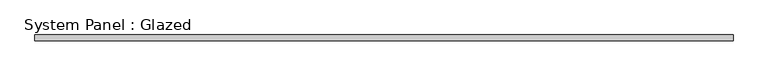
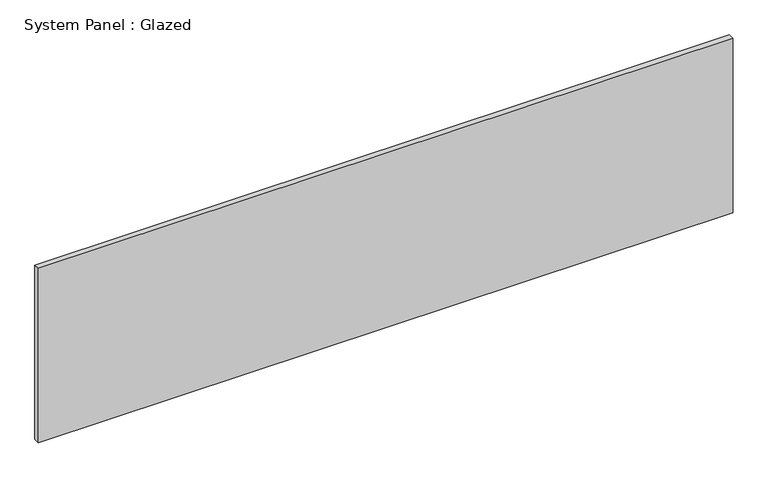
"""IFC4 building model written with IfcOpenShell, lengths in millimetres: plate geometry, System Panel : Glazed."""

import ifcopenshell
import ifcopenshell.guid

model = None  # the IFC model being written
_history = None  # IfcOwnerHistory: only IFC2X3 demands one
_inside = {}  # id of a spatial element -> (the spatial element, [elements in it])
_under = {}  # id of a project, library or spatial element -> (it, [spatial elements below it])
_declared = {}  # id of a project -> (the project, [libraries it declares])
_typed = {}  # id of a type object -> (the type object, [elements of that type])
_made_of = {}  # id of a material, layer set ... -> (it, [elements and type objects made of it])


def new_model(schema):
    """Start an empty IFC model of exactly this schema.

    Asked for "IFC4X3", IfcOpenShell would pick the latest addendum, in which some entities
    have other attributes; the version numbers below select the first issue.
    IFC2X3 requires an IfcOwnerHistory on every rooted entity: one is made here for all.
    """
    global model, _history
    if schema == "IFC4X3":
        model = ifcopenshell.file(schema_version=(4, 3, 0, 0))
    else:
        model = ifcopenshell.file(schema=schema)
    _inside.clear()
    _under.clear()
    _declared.clear()
    _typed.clear()
    _made_of.clear()
    _history = None
    if model.schema == "IFC2X3":
        org = make("IfcOrganization", Name="unknown")
        user = make(
            "IfcPersonAndOrganization",
            ThePerson=make("IfcPerson", FamilyName="unknown"),
            TheOrganization=org,
        )
        app = make(
            "IfcApplication",
            ApplicationDeveloper=org,
            Version="unknown",
            ApplicationFullName="unknown",
            ApplicationIdentifier="unknown",
        )
        _history = make(
            "IfcOwnerHistory",
            OwningUser=user,
            OwningApplication=app,
            ChangeAction="ADDED",
            CreationDate=0,
        )
    return model


def make(cls, **values):
    """One entity of the class cls with the attributes given. An attribute that is None is left unset."""
    return model.create_entity(
        cls, **{name: value for name, value in values.items() if value is not None}
    )


def rooted(cls, **values):
    """An entity with a GlobalId (a new one), such as an element, a storey or a relation."""
    return make(cls, GlobalId=ifcopenshell.guid.new(), OwnerHistory=_history, **values)


def si_unit(unit_type, name, prefix=None):
    """IfcSIUnit, for example si_unit("LENGTHUNIT", "METRE", prefix="MILLI")."""
    return make("IfcSIUnit", UnitType=unit_type, Prefix=prefix, Name=name)


def assignment(units):
    """IfcUnitAssignment: the units of a project."""
    return None if units is None else make("IfcUnitAssignment", Units=units)


def point(xyz):
    """IfcCartesianPoint."""
    return None if xyz is None else make("IfcCartesianPoint", Coordinates=xyz)


def direction(xyz):
    """IfcDirection."""
    return None if xyz is None else make("IfcDirection", DirectionRatios=xyz)


def frame(location, z_axis=None, x_axis=None):
    """IfcAxis2Placement3D, a coordinate frame: its origin and axes. An axis left out is left unset."""
    return make(
        "IfcAxis2Placement3D",
        Location=point(location),
        Axis=direction(z_axis),
        RefDirection=direction(x_axis),
    )


def origin():
    """The frame at (0, 0, 0) with its axes left unset."""
    return frame((0.0, 0.0, 0.0))


def origin_with_axes():
    """The frame at (0, 0, 0) with the z axis (0, 0, 1) and the x axis (1, 0, 0) written out."""
    return frame((0.0, 0.0, 0.0), z_axis=(0.0, 0.0, 1.0), x_axis=(1.0, 0.0, 0.0))


def place(relative_to, where):
    """IfcLocalPlacement: puts the frame where relative to a parent placement (None: the world)."""
    return make(
        "IfcLocalPlacement", PlacementRelTo=relative_to, RelativePlacement=where
    )


def context(
    kind, dimensions, precision=None, world=None, true_north=None, identifier=None
):
    """IfcGeometricRepresentationContext, for example the 3D "Model" context."""
    return make(
        "IfcGeometricRepresentationContext",
        ContextIdentifier=identifier,
        ContextType=kind,
        CoordinateSpaceDimension=dimensions,
        Precision=precision,
        WorldCoordinateSystem=world,
        TrueNorth=true_north,
    )


def project(units=None, contexts=None):
    """IfcProject with its units and contexts."""
    return rooted(
        "IfcProject",
        Name="project",
        RepresentationContexts=contexts,
        UnitsInContext=assignment(units),
    )


def spatial(cls, under=None, at=None, **own):
    """A site, building, storey or space (cls), placed at a placement, below another one or the project."""
    s = rooted(cls, ObjectPlacement=at, **own)
    if under is not None:
        _under.setdefault(under.id(), (under, []))[1].append(s)
    return s


def polyline(points):
    """IfcPolyline through the points."""
    return make("IfcPolyline", Points=[point(p) for p in points])


def outline(outer, holes=None, kind="AREA"):
    """IfcArbitraryClosedProfileDef: a profile drawn as a closed curve; with holes, ...WithVoids."""
    if holes is None:
        return make("IfcArbitraryClosedProfileDef", ProfileType=kind, OuterCurve=outer)
    return make(
        "IfcArbitraryProfileDefWithVoids",
        ProfileType=kind,
        OuterCurve=outer,
        InnerCurves=holes,
    )


def extrude(swept, where, along, depth):
    """IfcExtrudedAreaSolid: the profile swept, set in the frame where, extruded along a direction by depth."""
    return make(
        "IfcExtrudedAreaSolid",
        SweptArea=swept,
        Position=where,
        ExtrudedDirection=direction(along),
        Depth=depth,
    )


def shape(context_of_items, identifier, shape_type, items):
    """IfcShapeRepresentation: the items that make up one representation, for example the "Body"."""
    return make(
        "IfcShapeRepresentation",
        ContextOfItems=context_of_items,
        RepresentationIdentifier=identifier,
        RepresentationType=shape_type,
        Items=items,
    )


def source(mapping_origin, context_of_items, identifier, shape_type, items):
    """IfcRepresentationMap: a shape defined once, which mapped items show again and again."""
    return make(
        "IfcRepresentationMap",
        MappingOrigin=mapping_origin,
        MappedRepresentation=shape(context_of_items, identifier, shape_type, items),
    )


def transform(
    local_origin,
    x_axis=None,
    y_axis=None,
    z_axis=None,
    scale=None,
    scale2=None,
    scale3=None,
    uniform=True,
):
    """IfcCartesianTransformationOperator3D, or its non-uniform kind. x_axis, y_axis, z_axis: its Axis1, 2, 3."""
    if uniform:
        return make(
            "IfcCartesianTransformationOperator3D",
            Axis1=direction(x_axis),
            Axis2=direction(y_axis),
            LocalOrigin=point(local_origin),
            Scale=scale,
            Axis3=direction(z_axis),
        )
    return make(
        "IfcCartesianTransformationOperator3DnonUniform",
        Axis1=direction(x_axis),
        Axis2=direction(y_axis),
        LocalOrigin=point(local_origin),
        Scale=scale,
        Axis3=direction(z_axis),
        Scale2=scale2,
        Scale3=scale3,
    )


def mapped(mapping_source, mapping_target):
    """IfcMappedItem: shows the shape of a source again, moved by a transform."""
    return make(
        "IfcMappedItem", MappingSource=mapping_source, MappingTarget=mapping_target
    )


def made_of(thing, what):
    """Note that an element or type object is made of a material, layer set ...; save() writes the relation."""
    if what is not None:
        _made_of.setdefault(what.id(), (what, []))[1].append(thing)
    return thing


def element(
    cls,
    number,
    at=None,
    inside=None,
    cuts=None,
    type_object=None,
    material=None,
    context=None,
    identifier="Body",
    shape_type=None,
    held_by="IfcProductDefinitionShape",
    body=None,
    shapes=None,
    **own,
):
    """One element of the class cls, such as IfcWall. Its Tag is "e" and its number.

    at: its placement. inside: the storey or other place that contains it. cuts: it is an
    opening in that element (IfcRelVoidsElement). A single representation is given by context,
    identifier, shape_type and body (its items); several are given by shapes. held_by: the class
    of the entity that holds the representations. save() writes the other relations.
    """
    e = rooted(cls, Tag="e%d" % number, ObjectPlacement=at, **own)
    if body is not None:
        shapes = [shape(context, identifier, shape_type, body)]
    if shapes is not None:
        e.Representation = make(held_by, Representations=shapes)
    if inside is not None:
        _inside.setdefault(inside.id(), (inside, []))[1].append(e)
    if cuts is not None:
        rooted(
            "IfcRelVoidsElement", RelatingBuildingElement=cuts, RelatedOpeningElement=e
        )
    if type_object is not None:
        _typed.setdefault(type_object.id(), (type_object, []))[1].append(e)
    return made_of(e, material)


def aggregate(whole, parts):
    """IfcRelAggregates: a whole, such as a stair, and the parts it consists of."""
    return rooted("IfcRelAggregates", RelatingObject=whole, RelatedObjects=parts)


def save(model, path):
    """Write the relations noted so far, then the file.

    IfcRelAggregates (storeys below a building ...), IfcRelContainedInSpatialStructure (elements
    in a storey), IfcRelDefinesByType, IfcRelAssociatesMaterial and IfcRelDeclares: one each for
    every whole, place, type object, material and project.
    """
    for whole, parts in _under.values():
        aggregate(whole, parts)
    for where, things in _inside.values():
        rooted(
            "IfcRelContainedInSpatialStructure",
            RelatedElements=things,
            RelatingStructure=where,
        )
    for kind, things in _typed.values():
        rooted("IfcRelDefinesByType", RelatedObjects=things, RelatingType=kind)
    for what, things in _made_of.values():
        rooted("IfcRelAssociatesMaterial", RelatedObjects=things, RelatingMaterial=what)
    for by, libraries in _declared.values():
        rooted("IfcRelDeclares", RelatingContext=by, RelatedDefinitions=libraries)
    model.write(path)


def system_panel_glazed_b70978ba(model_context):
    return source(origin(), model_context, "Body", "SweptSolid", [
        extrude(outline(polyline([(1543.05, -44.45), (-1543.05, -44.45), (-1543.05, -19.05), (1543.05, -19.05), (1543.05, -44.45)])), origin_with_axes(), (0.0, 0.0, 1.0), 819.15),
    ])


if __name__ == "__main__":
    model = new_model("IFC4")
    model_context = context("Model", 3, world=origin())
    ifc_project = project(units=[si_unit("LENGTHUNIT", "METRE", prefix="MILLI")], contexts=[model_context])
    site = spatial("IfcSite", under=ifc_project)
    building = spatial("IfcBuilding", under=site)
    placement = place(None, origin())
    system_panel_glazed_shape = system_panel_glazed_b70978ba(model_context)
    element("IfcPlate", 1, ObjectType="System Panel : Glazed", at=placement, inside=building, context=model_context, shape_type="MappedRepresentation", body=[
        mapped(system_panel_glazed_shape, transform((0.0, 0.0, 0.0), x_axis=(1.0, 0.0, 0.0), y_axis=(0.0, 1.0, 0.0), z_axis=(0.0, 0.0, 1.0))),
    ])
    save(model, "model.ifc")

# Revit data of these elements
# Type "System Panel : Glazed"
#   Construction Type Id = "GSP4R"
#   Analytic Construction = "1/8 in Pilkington single glazing"
#   Visual Light Transmittance = 0.9
#   Solar Heat Gain Coefficient = 0.86
#   Heat Transfer Coefficient (U) = 1.18115 BTU/(h·ft²·°F)
#   Define Thermal Properties by = 1
# Element 1 (IfcPlate, "System Panel : Glazed")
#   Materials on its faces: "Glass"
# Materials
#   "Glass": class "Glass", colour RGB 0 128 192, transparency 0.75, Description = "Soda Lime Glass", Cost = 0
